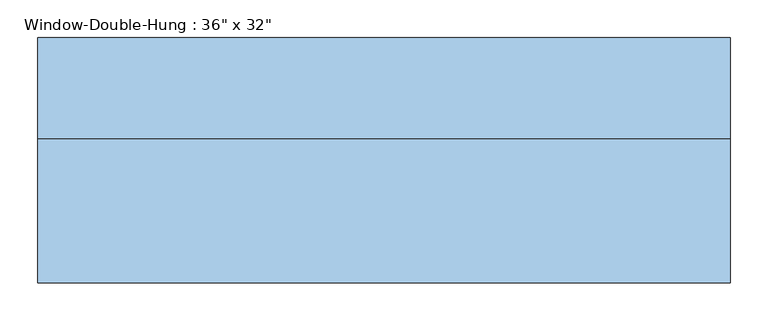
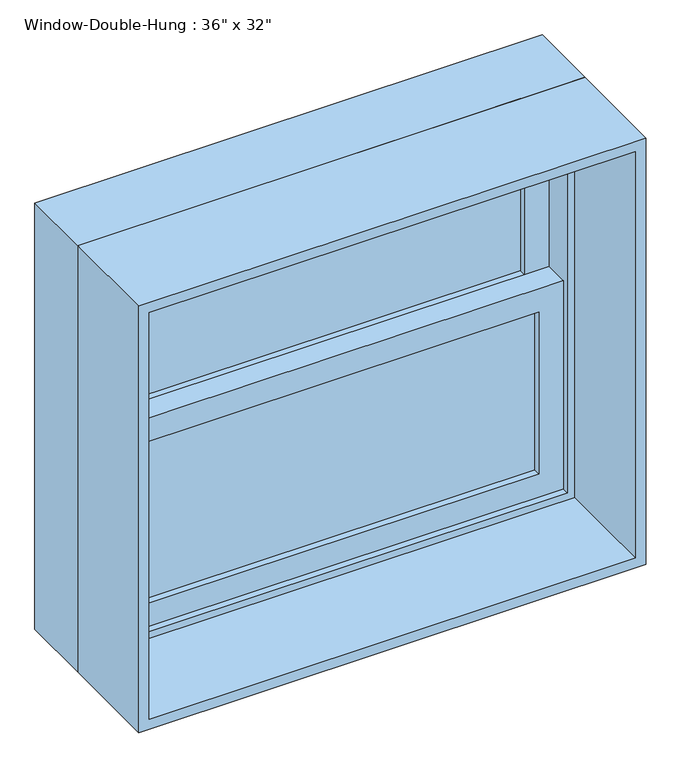
"""IFC4 building model written with IfcOpenShell, lengths in millimetres: window geometry."""

import ifcopenshell
import ifcopenshell.guid

model = None  # the IFC model being written
_history = None  # IfcOwnerHistory: only IFC2X3 demands one
_inside = {}  # id of a spatial element -> (the spatial element, [elements in it])
_under = {}  # id of a project, library or spatial element -> (it, [spatial elements below it])
_declared = {}  # id of a project -> (the project, [libraries it declares])
_typed = {}  # id of a type object -> (the type object, [elements of that type])
_made_of = {}  # id of a material, layer set ... -> (it, [elements and type objects made of it])


def new_model(schema):
    """Start an empty IFC model of exactly this schema.

    Asked for "IFC4X3", IfcOpenShell would pick the latest addendum, in which some entities
    have other attributes; the version numbers below select the first issue.
    IFC2X3 requires an IfcOwnerHistory on every rooted entity: one is made here for all.
    """
    global model, _history
    if schema == "IFC4X3":
        model = ifcopenshell.file(schema_version=(4, 3, 0, 0))
    else:
        model = ifcopenshell.file(schema=schema)
    _inside.clear()
    _under.clear()
    _declared.clear()
    _typed.clear()
    _made_of.clear()
    _history = None
    if model.schema == "IFC2X3":
        org = make("IfcOrganization", Name="unknown")
        user = make(
            "IfcPersonAndOrganization",
            ThePerson=make("IfcPerson", FamilyName="unknown"),
            TheOrganization=org,
        )
        app = make(
            "IfcApplication",
            ApplicationDeveloper=org,
            Version="unknown",
            ApplicationFullName="unknown",
            ApplicationIdentifier="unknown",
        )
        _history = make(
            "IfcOwnerHistory",
            OwningUser=user,
            OwningApplication=app,
            ChangeAction="ADDED",
            CreationDate=0,
        )
    return model


def make(cls, **values):
    """One entity of the class cls with the attributes given. An attribute that is None is left unset."""
    return model.create_entity(
        cls, **{name: value for name, value in values.items() if value is not None}
    )


def rooted(cls, **values):
    """An entity with a GlobalId (a new one), such as an element, a storey or a relation."""
    return make(cls, GlobalId=ifcopenshell.guid.new(), OwnerHistory=_history, **values)


def si_unit(unit_type, name, prefix=None):
    """IfcSIUnit, for example si_unit("LENGTHUNIT", "METRE", prefix="MILLI")."""
    return make("IfcSIUnit", UnitType=unit_type, Prefix=prefix, Name=name)


def assignment(units):
    """IfcUnitAssignment: the units of a project."""
    return None if units is None else make("IfcUnitAssignment", Units=units)


def point(xyz):
    """IfcCartesianPoint."""
    return None if xyz is None else make("IfcCartesianPoint", Coordinates=xyz)


def direction(xyz):
    """IfcDirection."""
    return None if xyz is None else make("IfcDirection", DirectionRatios=xyz)


def frame(location, z_axis=None, x_axis=None):
    """IfcAxis2Placement3D, a coordinate frame: its origin and axes. An axis left out is left unset."""
    return make(
        "IfcAxis2Placement3D",
        Location=point(location),
        Axis=direction(z_axis),
        RefDirection=direction(x_axis),
    )


def origin():
    """The frame at (0, 0, 0) with its axes left unset."""
    return frame((0.0, 0.0, 0.0))


def place(relative_to, where):
    """IfcLocalPlacement: puts the frame where relative to a parent placement (None: the world)."""
    return make(
        "IfcLocalPlacement", PlacementRelTo=relative_to, RelativePlacement=where
    )


def context(
    kind, dimensions, precision=None, world=None, true_north=None, identifier=None
):
    """IfcGeometricRepresentationContext, for example the 3D "Model" context."""
    return make(
        "IfcGeometricRepresentationContext",
        ContextIdentifier=identifier,
        ContextType=kind,
        CoordinateSpaceDimension=dimensions,
        Precision=precision,
        WorldCoordinateSystem=world,
        TrueNorth=true_north,
    )


def project(units=None, contexts=None):
    """IfcProject with its units and contexts."""
    return rooted(
        "IfcProject",
        Name="project",
        RepresentationContexts=contexts,
        UnitsInContext=assignment(units),
    )


def spatial(cls, under=None, at=None, **own):
    """A site, building, storey or space (cls), placed at a placement, below another one or the project."""
    s = rooted(cls, ObjectPlacement=at, **own)
    if under is not None:
        _under.setdefault(under.id(), (under, []))[1].append(s)
    return s


def polyline(points):
    """IfcPolyline through the points."""
    return make("IfcPolyline", Points=[point(p) for p in points])


def outline(outer, holes=None, kind="AREA"):
    """IfcArbitraryClosedProfileDef: a profile drawn as a closed curve; with holes, ...WithVoids."""
    if holes is None:
        return make("IfcArbitraryClosedProfileDef", ProfileType=kind, OuterCurve=outer)
    return make(
        "IfcArbitraryProfileDefWithVoids",
        ProfileType=kind,
        OuterCurve=outer,
        InnerCurves=holes,
    )


def extrude(swept, where, along, depth):
    """IfcExtrudedAreaSolid: the profile swept, set in the frame where, extruded along a direction by depth."""
    return make(
        "IfcExtrudedAreaSolid",
        SweptArea=swept,
        Position=where,
        ExtrudedDirection=direction(along),
        Depth=depth,
    )


def shape(context_of_items, identifier, shape_type, items):
    """IfcShapeRepresentation: the items that make up one representation, for example the "Body"."""
    return make(
        "IfcShapeRepresentation",
        ContextOfItems=context_of_items,
        RepresentationIdentifier=identifier,
        RepresentationType=shape_type,
        Items=items,
    )


def source(mapping_origin, context_of_items, identifier, shape_type, items):
    """IfcRepresentationMap: a shape defined once, which mapped items show again and again."""
    return make(
        "IfcRepresentationMap",
        MappingOrigin=mapping_origin,
        MappedRepresentation=shape(context_of_items, identifier, shape_type, items),
    )


def transform(
    local_origin,
    x_axis=None,
    y_axis=None,
    z_axis=None,
    scale=None,
    scale2=None,
    scale3=None,
    uniform=True,
):
    """IfcCartesianTransformationOperator3D, or its non-uniform kind. x_axis, y_axis, z_axis: its Axis1, 2, 3."""
    if uniform:
        return make(
            "IfcCartesianTransformationOperator3D",
            Axis1=direction(x_axis),
            Axis2=direction(y_axis),
            LocalOrigin=point(local_origin),
            Scale=scale,
            Axis3=direction(z_axis),
        )
    return make(
        "IfcCartesianTransformationOperator3DnonUniform",
        Axis1=direction(x_axis),
        Axis2=direction(y_axis),
        LocalOrigin=point(local_origin),
        Scale=scale,
        Axis3=direction(z_axis),
        Scale2=scale2,
        Scale3=scale3,
    )


def mapped(mapping_source, mapping_target):
    """IfcMappedItem: shows the shape of a source again, moved by a transform."""
    return make(
        "IfcMappedItem", MappingSource=mapping_source, MappingTarget=mapping_target
    )


def made_of(thing, what):
    """Note that an element or type object is made of a material, layer set ...; save() writes the relation."""
    if what is not None:
        _made_of.setdefault(what.id(), (what, []))[1].append(thing)
    return thing


def element(
    cls,
    number,
    at=None,
    inside=None,
    cuts=None,
    type_object=None,
    material=None,
    context=None,
    identifier="Body",
    shape_type=None,
    held_by="IfcProductDefinitionShape",
    body=None,
    shapes=None,
    **own,
):
    """One element of the class cls, such as IfcWall. Its Tag is "e" and its number.

    at: its placement. inside: the storey or other place that contains it. cuts: it is an
    opening in that element (IfcRelVoidsElement). A single representation is given by context,
    identifier, shape_type and body (its items); several are given by shapes. held_by: the class
    of the entity that holds the representations. save() writes the other relations.
    """
    e = rooted(cls, Tag="e%d" % number, ObjectPlacement=at, **own)
    if body is not None:
        shapes = [shape(context, identifier, shape_type, body)]
    if shapes is not None:
        e.Representation = make(held_by, Representations=shapes)
    if inside is not None:
        _inside.setdefault(inside.id(), (inside, []))[1].append(e)
    if cuts is not None:
        rooted(
            "IfcRelVoidsElement", RelatingBuildingElement=cuts, RelatedOpeningElement=e
        )
    if type_object is not None:
        _typed.setdefault(type_object.id(), (type_object, []))[1].append(e)
    return made_of(e, material)


def aggregate(whole, parts):
    """IfcRelAggregates: a whole, such as a stair, and the parts it consists of."""
    return rooted("IfcRelAggregates", RelatingObject=whole, RelatedObjects=parts)


def save(model, path):
    """Write the relations noted so far, then the file.

    IfcRelAggregates (storeys below a building ...), IfcRelContainedInSpatialStructure (elements
    in a storey), IfcRelDefinesByType, IfcRelAssociatesMaterial and IfcRelDeclares: one each for
    every whole, place, type object, material and project.
    """
    for whole, parts in _under.values():
        aggregate(whole, parts)
    for where, things in _inside.values():
        rooted(
            "IfcRelContainedInSpatialStructure",
            RelatedElements=things,
            RelatingStructure=where,
        )
    for kind, things in _typed.values():
        rooted("IfcRelDefinesByType", RelatedObjects=things, RelatingType=kind)
    for what, things in _made_of.values():
        rooted("IfcRelAssociatesMaterial", RelatedObjects=things, RelatingMaterial=what)
    for by, libraries in _declared.values():
        rooted("IfcRelDeclares", RelatingContext=by, RelatedDefinitions=libraries)
    model.write(path)


def window_e3cc3ff6(model_context):
    return source(origin(), model_context, "Body", "SweptSolid", [
        extrude(outline(polyline([(381.0, 82.55), (381.0, 76.2), (-381.0, 76.2), (-381.0, 82.55), (381.0, 82.55)])), frame((0.0, 0.0, 990.6), z_axis=(0.0, 0.0, 1.0), x_axis=(1.0, 0.0, 0.0)), (0.0, 0.0, 1.0), 307.975),
        extrude(outline(polyline([(-381.0, 69.85), (381.0, 69.85), (381.0, 63.5), (-381.0, 63.5), (-381.0, 69.85)])), frame((0.0, 0.0, 990.6), z_axis=(0.0, 0.0, 1.0), x_axis=(1.0, 0.0, 0.0)), (0.0, 0.0, 1.0), 307.975),
        extrude(outline(polyline([(381.0, 127.0), (381.0, 120.65), (-381.0, 120.65), (-381.0, 127.0), (381.0, 127.0)])), frame((0.0, 0.0, 1343.025), z_axis=(0.0, 0.0, 1.0), x_axis=(1.0, 0.0, 0.0)), (0.0, 0.0, 1.0), 307.975),
        extrude(outline(polyline([(-381.0, 114.3), (381.0, 114.3), (381.0, 107.95), (-381.0, 107.95), (-381.0, 114.3)])), frame((0.0, 0.0, 1343.025), z_axis=(0.0, 0.0, 1.0), x_axis=(1.0, 0.0, 0.0)), (0.0, 0.0, 1.0), 307.975),
        extrude(outline(polyline([(1343.025, -425.45), (946.15, -425.45), (946.15, 425.45), (1343.025, 425.45), (1343.025, -425.45)]), holes=[polyline([(1298.575, 381.0), (990.6, 381.0), (990.6, -381.0), (1298.575, -381.0), (1298.575, 381.0)])]), frame((0.0, 50.8, 0.0), z_axis=(0.0, 1.0, 0.0), x_axis=(0.0, 0.0, 1.0)), (0.0, 0.0, 1.0), 44.45),
        extrude(outline(polyline([(1695.45, -425.45), (1298.575, -425.45), (1298.575, 425.45), (1695.45, 425.45), (1695.45, -425.45)]), holes=[polyline([(1651.0, 381.0), (1343.025, 381.0), (1343.025, -381.0), (1651.0, -381.0), (1651.0, 381.0)])]), frame((0.0, 95.25, 0.0), z_axis=(0.0, 1.0, 0.0), x_axis=(0.0, 0.0, 1.0)), (0.0, 0.0, 1.0), 44.45),
        extrude(outline(polyline([(1727.2, -457.2), (914.4, -457.2), (914.4, 457.2), (1727.2, 457.2), (1727.2, -457.2)]), holes=[polyline([(1695.45, 425.45), (946.15, 425.45), (946.15, -425.45), (1695.45, -425.45), (1695.45, 425.45)])]), frame((0.0, 38.1, 0.0), z_axis=(0.0, 1.0, 0.0), x_axis=(0.0, 0.0, 1.0)), (0.0, 0.0, 1.0), 133.35),
        extrude(outline(polyline([(1727.2, 457.2), (1727.2, -457.2), (914.4, -457.2), (914.4, 457.2), (1727.2, 457.2)]), holes=[polyline([(1708.15, 438.15), (933.45, 438.15), (933.45, -438.15), (1708.15, -438.15), (1708.15, 438.15)])]), frame((0.0, -152.4, 0.0), z_axis=(0.0, 1.0, 0.0), x_axis=(0.0, 0.0, 1.0)), (0.0, 0.0, 1.0), 190.5),
    ])


if __name__ == "__main__":
    model = new_model("IFC4")
    model_context = context("Model", 3, world=origin())
    ifc_project = project(units=[si_unit("LENGTHUNIT", "METRE", prefix="MILLI")], contexts=[model_context])
    site = spatial("IfcSite", under=ifc_project)
    building = spatial("IfcBuilding", under=site)
    placement = place(None, origin())
    window_shape = window_e3cc3ff6(model_context)
    element("IfcWindow", 1, ObjectType="Window-Double-Hung : 36\" x 32\"", at=placement, inside=building, context=model_context, shape_type="MappedRepresentation", body=[
        mapped(window_shape, transform((0.0, 0.0, 0.0), x_axis=(1.0, 0.0, 0.0), y_axis=(0.0, 1.0, 0.0), z_axis=(0.0, 0.0, 1.0))),
    ])
    save(model, "model.ifc")

# Revit data of these elements
# Type "Window-Double-Hung : 36\" x 32\""
#   Type Mark = "19"
#   Fire Rating = "0.5h"
#   Construction Type Id = "DG-DR"
#   Assembly Code = "B2020100"
#   Analytic Construction = "Double glazing - domestic"
#   Wall Thickness [instance default] = 0' - 6"
#   Window Inset [instance default] = 0' - 0"
#   Visual Light Transmittance = 0.81
#   Thermal Resistance (R) = 1.8146 (h·ft²·°F)/BTU
#   Solar Heat Gain Coefficient = 0.76
#   Muntin Width = 2' - 6"
#   Muntin Height = 1' - 0 1/8"
#   Interior Wall Closure [instance default] = 0' - 1 1/2"
#   Rough Width = 3' - 0 1/2"
#   Rough Height = 2' - 8 1/2"
#   Frame Extension [instance default] = 0' - 1 1/4"
#   Exterior Wall Closure [instance default] = 0' - 0 1/2"
#   Extension Jamb [instance default] = 0' - 1 1/2"
#   Heat Transfer Coefficient (U) = 0.5511 BTU/(h·ft²·°F)
#   Height = 2' - 8"
#   Width = 3' - 0"
#   Top Muntin Visibility = yes
#   Indicator Visibility [instance default] = yes
#   Extension Jamb Visibility [instance default] = yes
#   Interior Trim Visibility [instance default] = yes
#   Exterior Trim Visibility [instance default] = yes
#   Define Thermal Properties by = 1
#   Bottom Muntin Visibility = yes
#   Muntin Pattern = Muntin Pattern_2x2 : Muntin Pattern_2x2
#   Interior Trim Material = Wood - Stained
#   Interior Trim = Trim-Window-Interior-Flat : Picture Frame
#   Exterior Trim Material = Clad - White
#   Exterior Trim = Trim-Window-Exterior-Flat : with Sill
#   Glass Panel Material = Glass
#   Exterior Frame Material = Clad - White
#   Interior Frame Material = Wood - Stained
#   Wall Closure = (empty or 0)
# Element 1 (IfcWindow, "Window-Double-Hung : 36\" x 32\"")
#   Wall Thickness = 1' - 0"
#   Extension Jamb = 0' - 7 1/2"
#   Materials on its faces: "Wood - Stained", "Glass", "Clad - White"
# Materials
#   "Wood - Stained": class "Wood", colour RGB 224 178 126, transparency 0, Cost = 0
#   "Clad - White": class "Wood", colour RGB 242 242 238, transparency 0, Cost = 0
#   "Glass": class "Glass", colour RGB 0 128 192, transparency 0.75, Description = "Soda Lime Glass", Cost = 0
